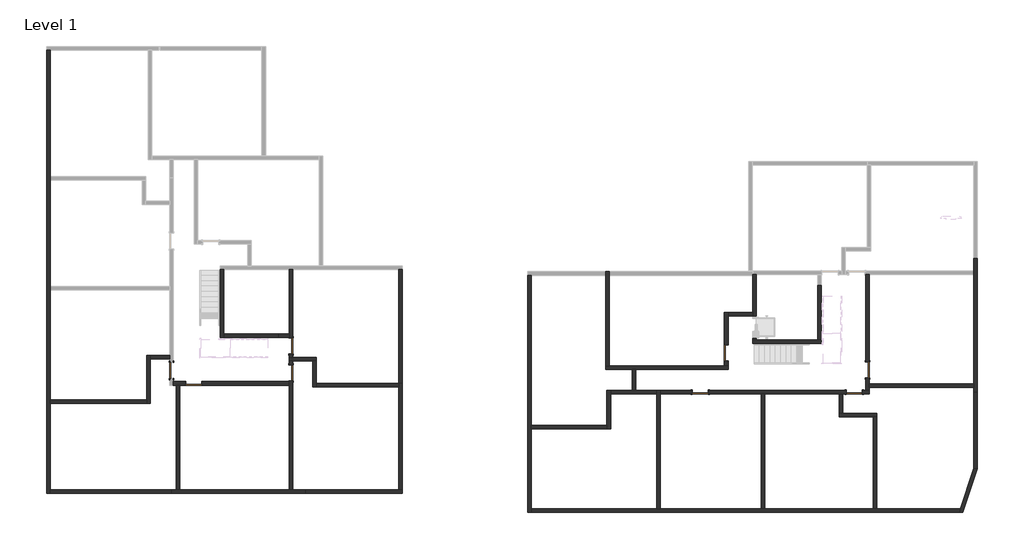
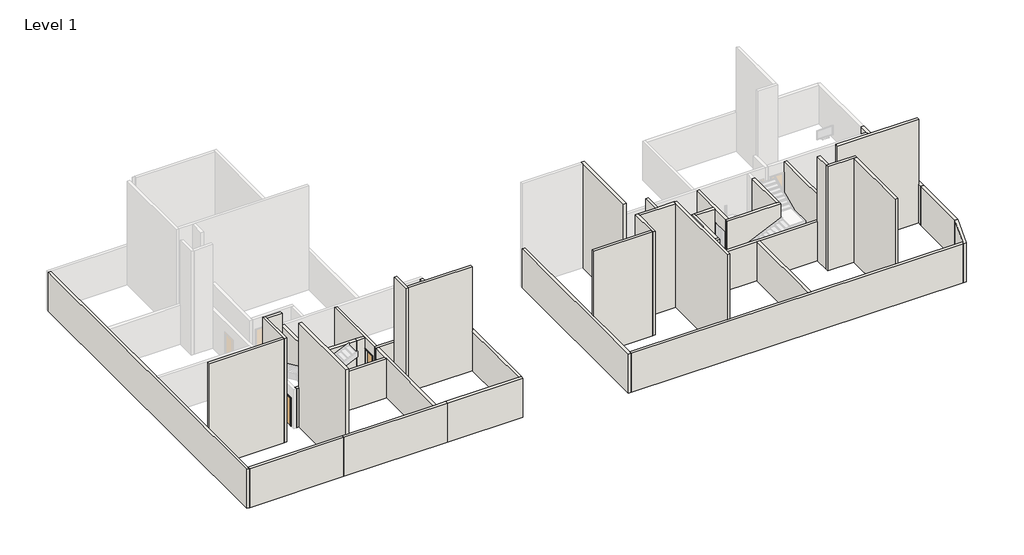
# One storey, part 1 of 2: 43 walls, 8 doors.
"""IFC4 building model written with IfcOpenShell, lengths in millimetres."""

import ifcopenshell
import ifcopenshell.guid

model = None  # the IFC model being written
_history = None  # IfcOwnerHistory: only IFC2X3 demands one
_inside = {}  # id of a spatial element -> (the spatial element, [elements in it])
_under = {}  # id of a project, library or spatial element -> (it, [spatial elements below it])
_declared = {}  # id of a project -> (the project, [libraries it declares])
_typed = {}  # id of a type object -> (the type object, [elements of that type])
_made_of = {}  # id of a material, layer set ... -> (it, [elements and type objects made of it])


def new_model(schema):
    """Start an empty IFC model of exactly this schema.

    Asked for "IFC4X3", IfcOpenShell would pick the latest addendum, in which some entities
    have other attributes; the version numbers below select the first issue.
    IFC2X3 requires an IfcOwnerHistory on every rooted entity: one is made here for all.
    """
    global model, _history
    if schema == "IFC4X3":
        model = ifcopenshell.file(schema_version=(4, 3, 0, 0))
    else:
        model = ifcopenshell.file(schema=schema)
    _inside.clear()
    _under.clear()
    _declared.clear()
    _typed.clear()
    _made_of.clear()
    _history = None
    if model.schema == "IFC2X3":
        org = make("IfcOrganization", Name="unknown")
        user = make(
            "IfcPersonAndOrganization",
            ThePerson=make("IfcPerson", FamilyName="unknown"),
            TheOrganization=org,
        )
        app = make(
            "IfcApplication",
            ApplicationDeveloper=org,
            Version="unknown",
            ApplicationFullName="unknown",
            ApplicationIdentifier="unknown",
        )
        _history = make(
            "IfcOwnerHistory",
            OwningUser=user,
            OwningApplication=app,
            ChangeAction="ADDED",
            CreationDate=0,
        )
    return model


def make(cls, **values):
    """One entity of the class cls with the attributes given. An attribute that is None is left unset."""
    return model.create_entity(
        cls, **{name: value for name, value in values.items() if value is not None}
    )


def rooted(cls, **values):
    """An entity with a GlobalId (a new one), such as an element, a storey or a relation."""
    return make(cls, GlobalId=ifcopenshell.guid.new(), OwnerHistory=_history, **values)


def si_unit(unit_type, name, prefix=None):
    """IfcSIUnit, for example si_unit("LENGTHUNIT", "METRE", prefix="MILLI")."""
    return make("IfcSIUnit", UnitType=unit_type, Prefix=prefix, Name=name)


def assignment(units):
    """IfcUnitAssignment: the units of a project."""
    return None if units is None else make("IfcUnitAssignment", Units=units)


def point(xyz):
    """IfcCartesianPoint."""
    return None if xyz is None else make("IfcCartesianPoint", Coordinates=xyz)


def direction(xyz):
    """IfcDirection."""
    return None if xyz is None else make("IfcDirection", DirectionRatios=xyz)


def frame(location, z_axis=None, x_axis=None):
    """IfcAxis2Placement3D, a coordinate frame: its origin and axes. An axis left out is left unset."""
    return make(
        "IfcAxis2Placement3D",
        Location=point(location),
        Axis=direction(z_axis),
        RefDirection=direction(x_axis),
    )


def origin():
    """The frame at (0, 0, 0) with its axes left unset."""
    return frame((0.0, 0.0, 0.0))


def origin_with_axes():
    """The frame at (0, 0, 0) with the z axis (0, 0, 1) and the x axis (1, 0, 0) written out."""
    return frame((0.0, 0.0, 0.0), z_axis=(0.0, 0.0, 1.0), x_axis=(1.0, 0.0, 0.0))


def place(relative_to, where):
    """IfcLocalPlacement: puts the frame where relative to a parent placement (None: the world)."""
    return make(
        "IfcLocalPlacement", PlacementRelTo=relative_to, RelativePlacement=where
    )


def context(
    kind, dimensions, precision=None, world=None, true_north=None, identifier=None
):
    """IfcGeometricRepresentationContext, for example the 3D "Model" context."""
    return make(
        "IfcGeometricRepresentationContext",
        ContextIdentifier=identifier,
        ContextType=kind,
        CoordinateSpaceDimension=dimensions,
        Precision=precision,
        WorldCoordinateSystem=world,
        TrueNorth=true_north,
    )


def project(units=None, contexts=None):
    """IfcProject with its units and contexts."""
    return rooted(
        "IfcProject",
        Name="project",
        RepresentationContexts=contexts,
        UnitsInContext=assignment(units),
    )


def spatial(cls, under=None, at=None, **own):
    """A site, building, storey or space (cls), placed at a placement, below another one or the project."""
    s = rooted(cls, ObjectPlacement=at, **own)
    if under is not None:
        _under.setdefault(under.id(), (under, []))[1].append(s)
    return s


def polyline(points):
    """IfcPolyline through the points."""
    return make("IfcPolyline", Points=[point(p) for p in points])


def outline(outer, holes=None, kind="AREA"):
    """IfcArbitraryClosedProfileDef: a profile drawn as a closed curve; with holes, ...WithVoids."""
    if holes is None:
        return make("IfcArbitraryClosedProfileDef", ProfileType=kind, OuterCurve=outer)
    return make(
        "IfcArbitraryProfileDefWithVoids",
        ProfileType=kind,
        OuterCurve=outer,
        InnerCurves=holes,
    )


def extrude(swept, where, along, depth):
    """IfcExtrudedAreaSolid: the profile swept, set in the frame where, extruded along a direction by depth."""
    return make(
        "IfcExtrudedAreaSolid",
        SweptArea=swept,
        Position=where,
        ExtrudedDirection=direction(along),
        Depth=depth,
    )


def faces_of(points, faces, orient=None, outer=None):
    """IfcFace entities. A face is a list of loops; a loop is a list of indices into points, from 0.

    orient and outer hold one flag for each loop. By default every Orientation is true, the
    first loop of a face is its IfcFaceOuterBound and the others are IfcFaceBound.
    """
    made = []
    for i, loops in enumerate(faces):
        bounds = []
        for j, loop in enumerate(loops):
            is_outer = j == 0 if outer is None else outer[i][j]
            bounds.append(
                make(
                    "IfcFaceOuterBound" if is_outer else "IfcFaceBound",
                    Bound=make("IfcPolyLoop", Polygon=[points[k] for k in loop]),
                    Orientation=True if orient is None else orient[i][j],
                )
            )
        made.append(make("IfcFace", Bounds=bounds))
    return made


def faceted_brep(points, faces, orient=None, outer=None, voids=None):
    """IfcFacetedBrep: a solid bounded by flat faces; with voids (closed shells), ...WithVoids."""
    shared = [point(p) for p in points]
    hull = make("IfcClosedShell", CfsFaces=faces_of(shared, faces, orient, outer))
    if voids is None:
        return make("IfcFacetedBrep", Outer=hull)
    return make(
        "IfcFacetedBrepWithVoids",
        Outer=hull,
        Voids=[
            make(cls, CfsFaces=faces_of(shared, fs, o, b)) for cls, fs, o, b in voids
        ],
    )


def shape(context_of_items, identifier, shape_type, items):
    """IfcShapeRepresentation: the items that make up one representation, for example the "Body"."""
    return make(
        "IfcShapeRepresentation",
        ContextOfItems=context_of_items,
        RepresentationIdentifier=identifier,
        RepresentationType=shape_type,
        Items=items,
    )


def source(mapping_origin, context_of_items, identifier, shape_type, items):
    """IfcRepresentationMap: a shape defined once, which mapped items show again and again."""
    return make(
        "IfcRepresentationMap",
        MappingOrigin=mapping_origin,
        MappedRepresentation=shape(context_of_items, identifier, shape_type, items),
    )


def transform(
    local_origin,
    x_axis=None,
    y_axis=None,
    z_axis=None,
    scale=None,
    scale2=None,
    scale3=None,
    uniform=True,
):
    """IfcCartesianTransformationOperator3D, or its non-uniform kind. x_axis, y_axis, z_axis: its Axis1, 2, 3."""
    if uniform:
        return make(
            "IfcCartesianTransformationOperator3D",
            Axis1=direction(x_axis),
            Axis2=direction(y_axis),
            LocalOrigin=point(local_origin),
            Scale=scale,
            Axis3=direction(z_axis),
        )
    return make(
        "IfcCartesianTransformationOperator3DnonUniform",
        Axis1=direction(x_axis),
        Axis2=direction(y_axis),
        LocalOrigin=point(local_origin),
        Scale=scale,
        Axis3=direction(z_axis),
        Scale2=scale2,
        Scale3=scale3,
    )


def mapped(mapping_source, mapping_target):
    """IfcMappedItem: shows the shape of a source again, moved by a transform."""
    return make(
        "IfcMappedItem", MappingSource=mapping_source, MappingTarget=mapping_target
    )


def made_of(thing, what):
    """Note that an element or type object is made of a material, layer set ...; save() writes the relation."""
    if what is not None:
        _made_of.setdefault(what.id(), (what, []))[1].append(thing)
    return thing


def element(
    cls,
    number,
    at=None,
    inside=None,
    cuts=None,
    type_object=None,
    material=None,
    context=None,
    identifier="Body",
    shape_type=None,
    held_by="IfcProductDefinitionShape",
    body=None,
    shapes=None,
    **own,
):
    """One element of the class cls, such as IfcWall. Its Tag is "e" and its number.

    at: its placement. inside: the storey or other place that contains it. cuts: it is an
    opening in that element (IfcRelVoidsElement). A single representation is given by context,
    identifier, shape_type and body (its items); several are given by shapes. held_by: the class
    of the entity that holds the representations. save() writes the other relations.
    """
    e = rooted(cls, Tag="e%d" % number, ObjectPlacement=at, **own)
    if body is not None:
        shapes = [shape(context, identifier, shape_type, body)]
    if shapes is not None:
        e.Representation = make(held_by, Representations=shapes)
    if inside is not None:
        _inside.setdefault(inside.id(), (inside, []))[1].append(e)
    if cuts is not None:
        rooted(
            "IfcRelVoidsElement", RelatingBuildingElement=cuts, RelatedOpeningElement=e
        )
    if type_object is not None:
        _typed.setdefault(type_object.id(), (type_object, []))[1].append(e)
    return made_of(e, material)


def aggregate(whole, parts):
    """IfcRelAggregates: a whole, such as a stair, and the parts it consists of."""
    return rooted("IfcRelAggregates", RelatingObject=whole, RelatedObjects=parts)


def save(model, path):
    """Write the relations noted so far, then the file.

    IfcRelAggregates (storeys below a building ...), IfcRelContainedInSpatialStructure (elements
    in a storey), IfcRelDefinesByType, IfcRelAssociatesMaterial and IfcRelDeclares: one each for
    every whole, place, type object, material and project.
    """
    for whole, parts in _under.values():
        aggregate(whole, parts)
    for where, things in _inside.values():
        rooted(
            "IfcRelContainedInSpatialStructure",
            RelatedElements=things,
            RelatingStructure=where,
        )
    for kind, things in _typed.values():
        rooted("IfcRelDefinesByType", RelatedObjects=things, RelatingType=kind)
    for what, things in _made_of.values():
        rooted("IfcRelAssociatesMaterial", RelatedObjects=things, RelatingMaterial=what)
    for by, libraries in _declared.values():
        rooted("IfcRelDeclares", RelatingContext=by, RelatedDefinitions=libraries)
    model.write(path)


def m_single_flush_0915_x_2134mm_727434cd(model_context):
    return source(origin(), model_context, "Body", "SweptSolid", [
        extrude(outline(polyline([(2210.0, -533.5), (0.0, -533.5), (0.0, -457.5), (2134.0, -457.5), (2134.0, 457.5), (0.0, 457.5), (0.0, 533.5), (2210.0, 533.5), (2210.0, -533.5)])), frame((0.0, -125.0, 0.0), z_axis=(0.0, 1.0, 0.0), x_axis=(0.0, 0.0, 1.0)), (0.0, 0.0, 1.0), 25.0),
        extrude(outline(polyline([(2210.0, 533.5), (2210.0, -533.5), (0.0, -533.5), (0.0, -457.5), (2134.0, -457.5), (2134.0, 457.5), (0.0, 457.5), (0.0, 533.5), (2210.0, 533.5)])), frame((0.0, 100.0, 0.0), z_axis=(0.0, 1.0, 0.0), x_axis=(0.0, 0.0, 1.0)), (0.0, 0.0, 1.0), 25.0),
        extrude(outline(polyline([(457.5, -49.0), (457.5, -100.0), (-457.5, -100.0), (-457.5, -49.0), (457.5, -49.0)])), origin_with_axes(), (0.0, 0.0, 1.0), 2134.0),
    ])


def m_single_flush_0915_x_2134mm_6a9e8738(model_context):
    return source(origin(), model_context, "Body", "SweptSolid", [
        extrude(outline(polyline([(2210.0, -533.5), (0.0, -533.5), (0.0, -457.5), (2134.0, -457.5), (2134.0, 457.5), (0.0, 457.5), (0.0, 533.5), (2210.0, 533.5), (2210.0, -533.5)])), frame((0.0, 100.0, 0.0), z_axis=(0.0, 1.0, 0.0), x_axis=(0.0, 0.0, 1.0)), (0.0, 0.0, 1.0), 25.0),
        extrude(outline(polyline([(2210.0, 533.5), (2210.0, -533.5), (0.0, -533.5), (0.0, -457.5), (2134.0, -457.5), (2134.0, 457.5), (0.0, 457.5), (0.0, 533.5), (2210.0, 533.5)])), frame((0.0, -125.0, 0.0), z_axis=(0.0, 1.0, 0.0), x_axis=(0.0, 0.0, 1.0)), (0.0, 0.0, 1.0), 25.0),
        extrude(outline(polyline([(457.5, 49.0), (-457.5, 49.0), (-457.5, 100.0), (457.5, 100.0), (457.5, 49.0)])), origin_with_axes(), (0.0, 0.0, 1.0), 2134.0),
    ])


model = new_model("IFC4")

# Units and contexts
model_context = context("Model", 3, world=origin())
ifc_project = project(units=[si_unit("LENGTHUNIT", "METRE", prefix="MILLI")], contexts=[model_context])

# Site, building, storey
site = spatial("IfcSite", under=ifc_project)
building = spatial("IfcBuilding", under=site)
storey = spatial("IfcBuildingStorey", under=building, Name="Level 1", Elevation=0.0)

# Doors
placement = place(None, origin())
m_single_flush_0915_x_2134mm_shape = m_single_flush_0915_x_2134mm_727434cd(model_context)
element("IfcDoor", 1, ObjectType="M_Single-Flush : 0915 x 2134mm", at=placement, inside=storey, context=model_context, shape_type="MappedRepresentation", body=[
    mapped(m_single_flush_0915_x_2134mm_shape, transform((16070.6041014, -3023.024372, 0.0), x_axis=(0.0, -1.0, 0.0), y_axis=(1.0, 0.0, 0.0), z_axis=(0.0, 0.0, 1.0))),
])
element("IfcDoor", 2, ObjectType="M_Single-Flush : 0915 x 2134mm", at=placement, inside=storey, context=model_context, shape_type="MappedRepresentation", body=[
    mapped(m_single_flush_0915_x_2134mm_shape, transform((-8530.3449834, -4137.6378151, 0.0), x_axis=(0.0, 1.0, 0.0), y_axis=(-1.0, 0.0, 0.0), z_axis=(0.0, 0.0, 1.0))),
])
m_single_flush_0915_x_2134mm_2_shape = m_single_flush_0915_x_2134mm_6a9e8738(model_context)
element("IfcDoor", 3, ObjectType="M_Single-Flush : 0915 x 2134mm", at=placement, inside=storey, context=model_context, shape_type="MappedRepresentation", body=[
    mapped(m_single_flush_0915_x_2134mm_2_shape, transform((14602.336337, -5240.0098119, 0.0), x_axis=(-1.0, 0.0, 0.0), y_axis=(0.0, -1.0, 0.0), z_axis=(0.0, 0.0, 1.0))),
])
element("IfcDoor", 4, ObjectType="M_Single-Flush : 0915 x 2134mm", at=placement, inside=storey, context=model_context, shape_type="MappedRepresentation", body=[
    mapped(m_single_flush_0915_x_2134mm_2_shape, transform((24048.8612349, -3982.5098119, 0.0), x_axis=(0.0, -1.0, 0.0), y_axis=(1.0, 0.0, 0.0), z_axis=(0.0, 0.0, 1.0))),
])
element("IfcDoor", 5, ObjectType="M_Single-Flush : 0915 x 2134mm", at=placement, inside=storey, context=model_context, shape_type="MappedRepresentation", body=[
    mapped(m_single_flush_0915_x_2134mm_2_shape, transform((23308.8612349, -5240.0098119, 0.0), x_axis=(-1.0, 0.0, 0.0), y_axis=(0.0, -1.0, 0.0), z_axis=(0.0, 0.0, 1.0))),
])
element("IfcDoor", 6, ObjectType="M_Single-Flush : 0915 x 2134mm", at=placement, inside=storey, context=model_context, shape_type="MappedRepresentation", body=[
    mapped(m_single_flush_0915_x_2134mm_2_shape, transform((-14032.3304233, -4739.1627129, 0.0), x_axis=(-1.0, 0.0, 0.0), y_axis=(0.0, -1.0, 0.0), z_axis=(0.0, 0.0, 1.0))),
])
element("IfcDoor", 7, ObjectType="M_Single-Flush : 0915 x 2134mm", at=placement, inside=storey, context=model_context, shape_type="MappedRepresentation", body=[
    mapped(m_single_flush_0915_x_2134mm_2_shape, transform((-8530.3449834, -2622.6378151, 0.0), x_axis=(0.0, -1.0, 0.0), y_axis=(1.0, 0.0, 0.0), z_axis=(0.0, 0.0, 1.0))),
])
element("IfcDoor", 8, ObjectType="M_Single-Flush : 0915 x 2134mm", at=placement, inside=storey, context=model_context, shape_type="MappedRepresentation", body=[
    mapped(m_single_flush_0915_x_2134mm_2_shape, transform((-15289.8304233, -3999.1627129, 0.0), x_axis=(0.0, 1.0, 0.0), y_axis=(-1.0, 0.0, 0.0), z_axis=(0.0, 0.0, 1.0))),
])

# Walls
element("IfcWall", 9, ObjectType="Generic - 200mm", at=placement, inside=storey, context=model_context, shape_type="Brep", body=[
    faceted_brep([(30068.8612349, 2319.475628, 0.0), (30068.8612349, 1619.475628, 0.0), (30068.8612349, 1419.475628, 0.0), (30068.8612349, -4760.0098119, 0.0), (30068.8612349, -4960.0098119, 0.0), (30068.8612349, -5240.0098119, 0.0), (30068.8612349, -5240.0098119, 3000.0), (30068.8612349, 1419.475628, 3000.0), (30068.8612349, 1619.475628, 3000.0), (30068.8612349, 2319.475628, 3000.0), (30268.8612349, 2319.475628, 0.0), (30268.8612349, 2319.475628, 3000.0), (30268.8612349, -5240.0098119, 3000.0), (30268.8612349, -5240.0098119, 0.0), (30268.3425199, 2319.475628, 0.0), (30069.3799498, -5240.0098119, 0.0), (30069.3799498, -5240.0098119, 3000.0), (30268.3425199, 2319.475628, 3000.0)], [[[0, 1, 2, 3, 4, 5, 6, 7, 8, 9]], [[10, 11, 12, 13]], [[5, 4, 3, 2, 1, 0, 14, 10, 13, 15]], [[6, 5, 15, 13, 12, 16]], [[9, 8, 7, 6, 16, 12, 11, 17]], [[0, 9, 17, 11, 10, 14]]]),
])
element("IfcWall", 10, ObjectType="Generic - 200mm", at=placement, inside=storey, context=model_context, shape_type="Brep", body=[
    faceted_brep([(30069.3799498, -5240.0098119, 0.0), (30069.3799498, -9543.0251929, 0.0), (30069.3799498, -9543.0251929, 3000.0), (30069.3799498, -5240.0098119, 3000.0), (30269.3799498, -5240.0098119, 0.0), (30269.3799498, -5240.0098119, 3000.0), (30269.3799498, -9575.863443, 3000.0), (30269.3799498, -9575.863443, 0.0), (30268.8612349, -5240.0098119, 0.0), (30268.8612349, -5240.0098119, 3000.0)], [[[0, 1, 2, 3]], [[4, 5, 6, 7]], [[1, 0, 8, 4, 7]], [[3, 2, 6, 5, 9]], [[0, 3, 9, 5, 4, 8]], [[2, 1, 7, 6]]]),
])
element("IfcWall", 11, ObjectType="Generic - 200mm", at=placement, inside=storey, context=model_context, shape_type="Brep", body=[
    faceted_brep([(21449.836337, -2276.2808257, 0.0), (21249.836337, -2276.2808257, 0.0), (17770.6041014, -2276.2808257, 0.0), (17570.6041014, -2276.2808257, 0.0), (17570.6041014, -2276.2808257, 3000.0), (17770.6041014, -2276.2808257, 3000.0), (21249.836337, -2276.2808257, 3000.0), (21449.836337, -2276.2808257, 3000.0), (21449.836337, -2476.2808257, 0.0), (21449.836337, -2476.2808257, 3000.0), (17570.6041014, -2476.2808257, 3000.0), (17570.6041014, -2476.2808257, 0.0)], [[[0, 1, 2, 3, 4, 5, 6, 7]], [[8, 9, 10, 11]], [[3, 2, 1, 0, 8, 11]], [[7, 6, 5, 4, 10, 9]], [[0, 7, 9, 8]], [[4, 3, 11, 10]]]),
])
element("IfcWall", 12, ObjectType="Generic - 200mm", at=placement, inside=storey, context=model_context, shape_type="SweptSolid", body=[
    extrude(outline(polyline([(18259.836337, -5340.0098119), (18259.836337, -11836.6907835), (18059.836337, -11836.6907835), (18059.836337, -5340.0098119), (18259.836337, -5340.0098119)])), origin_with_axes(), (0.0, 0.0, 1.0), 3000.0),
])
element("IfcWall", 13, ObjectType="Generic - 200mm", at=placement, inside=storey, context=model_context, shape_type="Brep", body=[
    faceted_brep([(29295.3124022, -11836.6907835, 0.0), (24588.8612349, -11836.6907835, 0.0), (24388.8612349, -11836.6907835, 0.0), (18259.836337, -11836.6907835, 0.0), (18059.836337, -11836.6907835, 0.0), (12342.1281129, -11836.6907835, 0.0), (12142.1281129, -11836.6907835, 0.0), (5043.716007, -11836.6907835, 0.0), (5043.716007, -11836.6907835, 3000.0), (18059.836337, -11836.6907835, 3000.0), (18259.836337, -11836.6907835, 3000.0), (29295.3124022, -11836.6907835, 3000.0), (29227.8162902, -12036.6907835, 0.0), (29227.8162902, -12036.6907835, 3000.0), (5043.716007, -12036.6907835, 3000.0), (5043.716007, -12036.6907835, 0.0)], [[[0, 1, 2, 3, 4, 5, 6, 7, 8, 9, 10, 11]], [[12, 13, 14, 15]], [[7, 6, 5, 4, 3, 2, 1, 0, 12, 15]], [[11, 10, 9, 8, 14, 13]], [[0, 11, 13, 12]], [[8, 7, 15, 14]]]),
])
element("IfcWall", 14, ObjectType="Generic - 200mm", at=placement, inside=storey, context=model_context, shape_type="Brep", body=[
    faceted_brep([(30069.3799498, -9543.0251929, 0.0), (29295.3124022, -11836.6907835, 0.0), (29227.8162902, -12036.6907835, 0.0), (29227.8162902, -12036.6907835, 3000.0), (29295.3124022, -11836.6907835, 3000.0), (30069.3799498, -9543.0251929, 3000.0), (30269.3799498, -9575.863443, 0.0), (30269.3799498, -9575.863443, 3000.0), (29438.8985612, -12036.6907835, 3000.0), (29438.8985612, -12036.6907835, 0.0)], [[[0, 1, 2, 3, 4, 5]], [[6, 7, 8, 9]], [[2, 1, 0, 6, 9]], [[5, 4, 3, 8, 7]], [[0, 5, 7, 6]], [[3, 2, 9, 8]]]),
])
element("IfcWall", 15, ObjectType="Generic - 200mm", at=placement, inside=storey, context=model_context, shape_type="Brep", body=[
    faceted_brep([(22851.3612349, -5140.0098119, 2134.0), (22851.3612349, -5140.0098119, 0.0), (15059.836337, -5140.0098119, 0.0), (15059.836337, -5140.0098119, 2134.0), (14144.836337, -5140.0098119, 2134.0), (14144.836337, -5140.0098119, 0.0), (12342.1281129, -5140.0098119, 0.0), (12342.1281129, -5140.0098119, 3000.0), (23948.8612349, -5140.0098119, 3000.0), (24148.8612349, -5140.0098119, 3000.0), (24163.3998354, -5140.0098119, 3000.0), (24163.3998354, -5140.0098119, 0.0), (24148.8612349, -5140.0098119, 0.0), (23948.8612349, -5140.0098119, 0.0), (23766.3612349, -5140.0098119, 0.0), (23766.3612349, -5140.0098119, 2134.0), (15059.836337, -5340.0098119, 0.0), (18059.836337, -5340.0098119, 0.0), (18259.836337, -5340.0098119, 0.0), (22468.8612349, -5340.0098119, 0.0), (22668.8612349, -5340.0098119, 0.0), (22851.3612349, -5340.0098119, 0.0), (22851.3612349, -5340.0098119, 2134.0), (23766.3612349, -5340.0098119, 2134.0), (23766.3612349, -5340.0098119, 0.0), (24163.3998354, -5340.0098119, 0.0), (24163.3998354, -5340.0098119, 3000.0), (18259.836337, -5340.0098119, 3000.0), (18059.836337, -5340.0098119, 3000.0), (12342.1281129, -5340.0098119, 3000.0), (12342.1281129, -5340.0098119, 0.0), (14144.836337, -5340.0098119, 0.0), (14144.836337, -5340.0098119, 2134.0), (15059.836337, -5340.0098119, 2134.0)], [[[0, 1, 2, 3, 4, 5, 6, 7, 8, 9, 10, 11, 12, 13, 14, 15]], [[16, 17, 18, 19, 20, 21, 22, 23, 24, 25, 26, 27, 28, 29, 30, 31, 32, 33]], [[30, 6, 5, 31]], [[2, 1, 21, 20, 19, 18, 17, 16]], [[14, 13, 12, 11, 25, 24]], [[10, 9, 8, 7, 29, 28, 27, 26]], [[11, 10, 26, 25]], [[4, 32, 31, 5]], [[33, 3, 2, 16]], [[3, 33, 32, 4]], [[22, 21, 1, 0]], [[23, 22, 0, 15]], [[24, 23, 15, 14]], [[7, 6, 30, 29]]]),
])
element("IfcWall", 16, ObjectType="Generic - 200mm", at=placement, inside=storey, context=model_context, shape_type="Brep", body=[
    faceted_brep([(4843.716007, 1379.9901881, 0.0), (4843.716007, -12036.6907835, 0.0), (4843.716007, -12036.6907835, 3000.0), (4843.716007, 1379.9901881, 3000.0), (5043.716007, 1379.9901881, 0.0), (5043.716007, 1379.9901881, 3000.0), (5043.716007, -11836.6907835, 3000.0), (5043.716007, -12036.6907835, 3000.0), (5043.716007, -12036.6907835, 0.0), (5043.716007, -11836.6907835, 0.0), (5043.716007, -7320.0098119, 0.0), (5043.716007, -7120.0098119, 0.0)], [[[0, 1, 2, 3]], [[4, 5, 6, 7, 8, 9, 10, 11]], [[1, 0, 4, 11, 10, 9, 8]], [[3, 2, 7, 6, 5]], [[2, 1, 8, 7]], [[0, 3, 5, 4]]]),
])
element("IfcWall", 17, ObjectType="Generic - 200mm", at=placement, inside=storey, context=model_context, shape_type="Brep", body=[
    faceted_brep([(24148.8612349, 1419.475628, 3000.0), (24148.8612349, -5140.0098119, 3000.0), (24148.8612349, -5140.0098119, 0.0), (24148.8612349, -4960.0098119, 0.0), (24148.8612349, -4760.0098119, 0.0), (24148.8612349, -4440.0098119, 0.0), (24148.8612349, -4440.0098119, 2134.0), (24148.8612349, -3525.0098119, 2134.0), (24148.8612349, -3525.0098119, 0.0), (24148.8612349, 1419.475628, 0.0), (23948.8612349, -5140.0098119, 3000.0), (23948.8612349, 1419.475628, 3000.0), (23948.8612349, 1419.475628, 0.0), (23948.8612349, -3525.0098119, 0.0), (23948.8612349, -3525.0098119, 2134.0), (23948.8612349, -4440.0098119, 2134.0), (23948.8612349, -4440.0098119, 0.0), (23948.8612349, -5140.0098119, 0.0)], [[[0, 1, 2, 3, 4, 5, 6, 7, 8, 9]], [[10, 11, 12, 13, 14, 15, 16, 17]], [[12, 9, 8, 13]], [[2, 17, 16, 5, 4, 3]], [[1, 0, 11, 10]], [[0, 9, 12, 11]], [[15, 6, 5, 16]], [[7, 14, 13, 8]], [[14, 7, 6, 15]], [[2, 1, 10, 17]]]),
])
element("IfcWall", 18, ObjectType="Generic - 200mm", at=placement, inside=storey, context=model_context, shape_type="SweptSolid", body=[
    extrude(outline(polyline([(21249.836337, -2276.2808257), (21249.836337, 799.475628), (21449.836337, 799.475628), (21449.836337, -2276.2808257), (21249.836337, -2276.2808257)])), origin_with_axes(), (0.0, 0.0, 1.0), 3000.0),
])
element("IfcWall", 19, ObjectType="Generic - 200mm", at=placement, inside=storey, context=model_context, shape_type="Brep", body=[
    faceted_brep([(17570.6041014, -2276.2808257, 3000.0), (17570.6041014, -920.524372, 3000.0), (17570.6041014, -720.524372, 3000.0), (17570.6041014, 1379.475628, 3000.0), (17570.6041014, 1419.475628, 3000.0), (17570.6041014, 1419.475628, 0.0), (17570.6041014, 1379.475628, 0.0), (17570.6041014, -720.524372, 0.0), (17570.6041014, -920.524372, 0.0), (17570.6041014, -926.2808257, 0.0), (17570.6041014, -926.2808257, 2000.0), (17570.6041014, -2181.2876228, 2000.0), (17570.6041014, -2181.2876228, 0.0), (17570.6041014, -2276.2808257, 0.0), (17770.6041014, 1419.475628, 3000.0), (17770.6041014, -2276.2808257, 3000.0), (17770.6041014, -2276.2808257, 0.0), (17770.6041014, -2181.2876228, 0.0), (17770.6041014, -2181.2876228, 2000.0), (17770.6041014, -926.2808257, 2000.0), (17770.6041014, -926.2808257, 0.0), (17770.6041014, 1419.475628, 0.0)], [[[0, 1, 2, 3, 4, 5, 6, 7, 8, 9, 10, 11, 12, 13]], [[14, 15, 16, 17, 18, 19, 20, 21]], [[16, 13, 12, 17]], [[5, 21, 20, 9, 8, 7, 6]], [[4, 3, 2, 1, 0, 15, 14]], [[0, 13, 16, 15]], [[5, 4, 14, 21]], [[11, 18, 17, 12]], [[19, 10, 9, 20]], [[10, 19, 18, 11]]]),
])
element("IfcWall", 20, ObjectType="Generic - 200mm", at=placement, inside=storey, context=model_context, shape_type="Brep", body=[
    faceted_brep([(9268.8612349, -3940.0098119, 0.0), (10768.8612349, -3940.0098119, 0.0), (10968.8612349, -3940.0098119, 0.0), (16170.6041014, -3940.0098119, 0.0), (16170.6041014, -3940.0098119, 3000.0), (9268.8612349, -3940.0098119, 3000.0), (9268.8612349, -3740.0098119, 0.0), (9268.8612349, -3740.0098119, 3000.0), (15970.6041014, -3740.0098119, 3000.0), (16170.6041014, -3740.0098119, 3000.0), (16170.6041014, -3740.0098119, 0.0), (15970.6041014, -3740.0098119, 0.0), (9468.8612349, -3740.0098119, 0.0)], [[[0, 1, 2, 3, 4, 5]], [[6, 7, 8, 9, 10, 11, 12]], [[3, 2, 1, 0, 6, 12, 11, 10]], [[5, 4, 9, 8, 7]], [[4, 3, 10, 9]], [[0, 5, 7, 6]]]),
])
element("IfcWall", 21, ObjectType="Generic - 200mm", at=placement, inside=storey, context=model_context, shape_type="Brep", body=[
    faceted_brep([(16170.6041014, -720.524372, 3000.0), (16170.6041014, -920.524372, 3000.0), (16170.6041014, -3740.0098119, 3000.0), (16170.6041014, -3740.0098119, 0.0), (16170.6041014, -3480.524372, 0.0), (16170.6041014, -3480.524372, 2134.0), (16170.6041014, -2565.524372, 2134.0), (16170.6041014, -2565.524372, 0.0), (16170.6041014, -920.524372, 0.0), (16170.6041014, -720.524372, 0.0), (15970.6041014, -3740.0098119, 3000.0), (15970.6041014, -720.524372, 3000.0), (15970.6041014, -720.524372, 0.0), (15970.6041014, -2565.524372, 0.0), (15970.6041014, -2565.524372, 2134.0), (15970.6041014, -3480.524372, 2134.0), (15970.6041014, -3480.524372, 0.0), (15970.6041014, -3740.0098119, 0.0)], [[[0, 1, 2, 3, 4, 5, 6, 7, 8, 9]], [[10, 11, 12, 13, 14, 15, 16, 17]], [[3, 17, 16, 4]], [[12, 9, 8, 7, 13]], [[2, 1, 0, 11, 10]], [[3, 2, 10, 17]], [[0, 9, 12, 11]], [[15, 5, 4, 16]], [[6, 14, 13, 7]], [[14, 6, 5, 15]]]),
])
element("IfcWall", 22, ObjectType="Generic - 200mm", at=placement, inside=storey, context=model_context, shape_type="SweptSolid", body=[
    extrude(outline(polyline([(17570.6041014, -920.524372), (16170.6041014, -920.524372), (16170.6041014, -720.524372), (17570.6041014, -720.524372), (17570.6041014, -920.524372)])), origin_with_axes(), (0.0, 0.0, 1.0), 3000.0),
])
element("IfcWall", 23, ObjectType="Generic - 200mm", at=placement, inside=storey, context=model_context, shape_type="Brep", body=[
    faceted_brep([(22468.8612349, -6641.2808257, 0.0), (24388.8612349, -6641.2808257, 0.0), (24588.8612349, -6641.2808257, 0.0), (24588.8612349, -6641.2808257, 8000.0), (24388.8612349, -6641.2808257, 8000.0), (22468.8612349, -6641.2808257, 8000.0), (22468.8612349, -6441.2808257, 0.0), (22468.8612349, -6441.2808257, 8000.0), (22668.8612349, -6441.2808257, 8000.0), (24588.8612349, -6441.2808257, 8000.0), (24588.8612349, -6441.2808257, 0.0), (22668.8612349, -6441.2808257, 0.0)], [[[0, 1, 2, 3, 4, 5]], [[6, 7, 8, 9, 10, 11]], [[2, 1, 0, 6, 11, 10]], [[5, 4, 3, 9, 8, 7]], [[3, 2, 10, 9]], [[0, 5, 7, 6]]]),
])
element("IfcWall", 24, ObjectType="Generic - 200mm", at=placement, inside=storey, context=model_context, shape_type="SweptSolid", body=[
    extrude(outline(polyline([(24388.8612349, -11836.6907835), (24388.8612349, -6641.2808257), (24588.8612349, -6641.2808257), (24588.8612349, -11836.6907835), (24388.8612349, -11836.6907835)])), origin_with_axes(), (0.0, 0.0, 1.0), 8000.0),
])
element("IfcWall", 25, ObjectType="Generic - 200mm", at=placement, inside=storey, context=model_context, shape_type="SweptSolid", body=[
    extrude(outline(polyline([(22668.8612349, -5340.0098119), (22668.8612349, -6441.2808257), (22468.8612349, -6441.2808257), (22468.8612349, -5340.0098119), (22668.8612349, -5340.0098119)])), origin_with_axes(), (0.0, 0.0, 1.0), 8000.0),
])
element("IfcWall", 26, ObjectType="Generic - 200mm", at=placement, inside=storey, context=model_context, shape_type="SweptSolid", body=[
    extrude(outline(polyline([(30068.8612349, -4960.0098119), (24148.8612349, -4960.0098119), (24148.8612349, -4760.0098119), (30068.8612349, -4760.0098119), (30068.8612349, -4960.0098119)])), origin_with_axes(), (0.0, 0.0, 1.0), 8000.0),
])
element("IfcWall", 27, ObjectType="Generic - 200mm", at=placement, inside=storey, context=model_context, shape_type="Brep", body=[
    faceted_brep([(9268.8612349, 1579.9901881, 0.0), (9268.8612349, 1379.9901881, 0.0), (9268.8612349, -3740.0098119, 0.0), (9268.8612349, -3740.0098119, 3000.0), (9268.8612349, -3740.0098119, 8000.0), (9268.8612349, 1379.9901881, 8000.0), (9268.8612349, 1579.9901881, 8000.0), (9468.8612349, 1579.9901881, 0.0), (9468.8612349, 1579.9901881, 8000.0), (9468.8612349, -3740.0098119, 8000.0), (9468.8612349, -3740.0098119, 0.0), (9468.8612349, 1379.475628, 0.0), (9468.8612349, 1579.475628, 0.0)], [[[0, 1, 2, 3, 4, 5, 6]], [[7, 8, 9, 10, 11, 12]], [[2, 1, 0, 7, 12, 11, 10]], [[6, 5, 4, 9, 8]], [[4, 3, 2, 10, 9]], [[0, 6, 8, 7]]]),
])
element("IfcWall", 28, ObjectType="Generic - 200mm", at=placement, inside=storey, context=model_context, shape_type="SweptSolid", body=[
    extrude(outline(polyline([(5043.716007, -7120.0098119), (9328.8612349, -7120.0098119), (9328.8612349, -7320.0098119), (5043.716007, -7320.0098119), (5043.716007, -7120.0098119)])), origin_with_axes(), (0.0, 0.0, 1.0), 8000.0),
])
element("IfcWall", 29, ObjectType="Generic - 200mm", at=placement, inside=storey, context=model_context, shape_type="Brep", body=[
    faceted_brep([(-2430.3449834, -4740.1378151, 0.0), (-2430.3449834, -4940.1378151, 0.0), (-2430.3449834, -10758.643998, 0.0), (-2430.3449834, -10758.643998, 3000.0), (-2430.3449834, -4740.1378151, 3000.0), (-2230.3449834, -4740.1378151, 0.0), (-2230.3449834, -4740.1378151, 3000.0), (-2230.3449834, -10758.643998, 3000.0), (-2230.3449834, -10758.643998, 0.0)], [[[0, 1, 2, 3, 4]], [[5, 6, 7, 8]], [[2, 1, 0, 5, 8]], [[4, 3, 7, 6]], [[3, 2, 8, 7]], [[0, 4, 6, 5]]]),
])
element("IfcWall", 30, ObjectType="Generic - 200mm", at=placement, inside=storey, context=model_context, shape_type="Brep", body=[
    faceted_brep([(-2230.3449834, -10758.643998, 0.0), (-2430.3449834, -10758.643998, 0.0), (-7730.3449834, -10758.643998, 0.0), (-7730.3449834, -10758.643998, 3000.0), (-2430.3449834, -10758.643998, 3000.0), (-2230.3449834, -10758.643998, 3000.0), (-2230.3449834, -10958.643998, 0.0), (-2230.3449834, -10958.643998, 3000.0), (-7730.3449834, -10958.643998, 3000.0), (-7730.3449834, -10958.643998, 0.0), (-7730.3449834, -10759.1627129, 0.0), (-7730.3449834, -10759.1627129, 3000.0)], [[[0, 1, 2, 3, 4, 5]], [[6, 7, 8, 9]], [[2, 1, 0, 6, 9, 10]], [[3, 2, 10, 9, 8, 11]], [[5, 4, 3, 11, 8, 7]], [[0, 5, 7, 6]]]),
])
element("IfcWall", 31, ObjectType="Generic - 200mm", at=placement, inside=storey, context=model_context, shape_type="Brep", body=[
    faceted_brep([(-7730.3449834, -10759.1627129, 0.0), (-8430.3449834, -10759.1627129, 0.0), (-8630.3449834, -10759.1627129, 0.0), (-14809.8304233, -10759.1627129, 0.0), (-15009.8304233, -10759.1627129, 0.0), (-15289.8304233, -10759.1627129, 0.0), (-15289.8304233, -10759.1627129, 3000.0), (-8630.3449834, -10759.1627129, 3000.0), (-8430.3449834, -10759.1627129, 3000.0), (-7730.3449834, -10759.1627129, 3000.0), (-7730.3449834, -10959.1627129, 0.0), (-7730.3449834, -10959.1627129, 3000.0), (-15289.8304233, -10959.1627129, 3000.0), (-15289.8304233, -10959.1627129, 0.0), (-7730.3449834, -10958.643998, 0.0), (-15289.8304233, -10759.6814279, 0.0), (-15289.8304233, -10759.6814279, 3000.0), (-7730.3449834, -10958.643998, 3000.0)], [[[0, 1, 2, 3, 4, 5, 6, 7, 8, 9]], [[10, 11, 12, 13]], [[5, 4, 3, 2, 1, 0, 14, 10, 13, 15]], [[6, 5, 15, 13, 12, 16]], [[9, 8, 7, 6, 16, 12, 11, 17]], [[0, 9, 17, 11, 10, 14]]]),
])
element("IfcWall", 32, ObjectType="Generic - 200mm", at=placement, inside=storey, context=model_context, shape_type="Brep", body=[
    faceted_brep([(-15289.8304233, -10759.6814279, 0.0), (-22146.5113948, -10759.6814279, 0.0), (-22146.5113948, -10759.6814279, 3000.0), (-15289.8304233, -10759.6814279, 3000.0), (-15289.8304233, -10959.6814279, 0.0), (-15289.8304233, -10959.6814279, 3000.0), (-22146.5113948, -10959.6814279, 3000.0), (-22146.5113948, -10959.6814279, 0.0), (-15289.8304233, -10959.1627129, 0.0), (-15289.8304233, -10959.1627129, 3000.0)], [[[0, 1, 2, 3]], [[4, 5, 6, 7]], [[1, 0, 8, 4, 7]], [[3, 2, 6, 5, 9]], [[0, 3, 9, 5, 4, 8]], [[2, 1, 7, 6]]]),
])
element("IfcWall", 33, ObjectType="Generic - 200mm", at=placement, inside=storey, context=model_context, shape_type="Brep", body=[
    faceted_brep([(-12326.101437, -2140.1378151, 0.0), (-12326.101437, -1940.1378151, 0.0), (-12326.101437, 1699.0944206, 0.0), (-12326.101437, 1699.0944206, 3000.0), (-12326.101437, -1940.1378151, 3000.0), (-12326.101437, -2140.1378151, 3000.0), (-12526.101437, -2140.1378151, 0.0), (-12526.101437, -2140.1378151, 3000.0), (-12526.101437, 1699.0944206, 3000.0), (-12526.101437, 1699.0944206, 0.0)], [[[0, 1, 2, 3, 4, 5]], [[6, 7, 8, 9]], [[2, 1, 0, 6, 9]], [[3, 2, 9, 8]], [[5, 4, 3, 8, 7]], [[0, 5, 7, 6]]]),
])
element("IfcWall", 34, ObjectType="Generic - 200mm", at=placement, inside=storey, context=model_context, shape_type="Brep", body=[
    faceted_brep([(-22146.5113948, -10959.6814279, 0.0), (-22146.5113948, -10759.6814279, 0.0), (-22146.5113948, -5879.1627129, 0.0), (-22146.5113948, -5679.1627129, 0.0), (-22146.5113948, 549.8621849, 0.0), (-22146.5113948, 749.8621849, 0.0), (-22146.5113948, 6769.8621849, 0.0), (-22146.5113948, 6969.8621849, 0.0), (-22146.5113948, 14109.8621849, 0.0), (-22146.5113948, 14109.8621849, 3000.0), (-22146.5113948, 6969.8621849, 3000.0), (-22146.5113948, 6769.8621849, 3000.0), (-22146.5113948, 749.8621849, 3000.0), (-22146.5113948, 549.8621849, 3000.0), (-22146.5113948, -10759.6814279, 3000.0), (-22146.5113948, -10959.6814279, 3000.0), (-22346.5113948, -10959.6814279, 0.0), (-22346.5113948, -10959.6814279, 3000.0), (-22346.5113948, 14109.8621849, 3000.0), (-22346.5113948, 14109.8621849, 0.0)], [[[0, 1, 2, 3, 4, 5, 6, 7, 8, 9, 10, 11, 12, 13, 14, 15]], [[16, 17, 18, 19]], [[8, 7, 6, 5, 4, 3, 2, 1, 0, 16, 19]], [[15, 14, 13, 12, 11, 10, 9, 18, 17]], [[9, 8, 19, 18]], [[0, 15, 17, 16]]]),
])
element("IfcWall", 35, ObjectType="Generic - 200mm", at=placement, inside=storey, context=model_context, shape_type="Brep", body=[
    faceted_brep([(-8630.3449834, -4839.1627129, 3000.0), (-15189.8304233, -4839.1627129, 3000.0), (-15189.8304233, -4839.1627129, 0.0), (-15009.8304233, -4839.1627129, 0.0), (-14809.8304233, -4839.1627129, 0.0), (-14489.8304233, -4839.1627129, 0.0), (-14489.8304233, -4839.1627129, 2134.0), (-13574.8304233, -4839.1627129, 2134.0), (-13574.8304233, -4839.1627129, 0.0), (-8630.3449834, -4839.1627129, 0.0), (-15189.8304233, -4639.1627129, 3000.0), (-8630.3449834, -4639.1627129, 3000.0), (-8630.3449834, -4639.1627129, 0.0), (-13574.8304233, -4639.1627129, 0.0), (-13574.8304233, -4639.1627129, 2134.0), (-14489.8304233, -4639.1627129, 2134.0), (-14489.8304233, -4639.1627129, 0.0), (-15189.8304233, -4639.1627129, 0.0)], [[[0, 1, 2, 3, 4, 5, 6, 7, 8, 9]], [[10, 11, 12, 13, 14, 15, 16, 17]], [[12, 9, 8, 13]], [[2, 17, 16, 5, 4, 3]], [[1, 0, 11, 10]], [[0, 9, 12, 11]], [[15, 6, 5, 16]], [[7, 14, 13, 8]], [[14, 7, 6, 15]], [[2, 1, 10, 17]]]),
])
element("IfcWall", 36, ObjectType="Generic - 200mm", at=placement, inside=storey, context=model_context, shape_type="SweptSolid", body=[
    extrude(outline(polyline([(-12326.101437, -1940.1378151), (-9250.3449834, -1940.1378151), (-9250.3449834, -2140.1378151), (-12326.101437, -2140.1378151), (-12326.101437, -1940.1378151)])), origin_with_axes(), (0.0, 0.0, 1.0), 3000.0),
])
element("IfcWall", 37, ObjectType="Generic - 200mm", at=placement, inside=storey, context=model_context, shape_type="SweptSolid", body=[
    extrude(outline(polyline([(-8630.3449834, -2140.1378151), (-9250.3449834, -2140.1378151), (-9250.3449834, -1940.1378151), (-8630.3449834, -1940.1378151), (-8630.3449834, -2140.1378151)])), origin_with_axes(), (0.0, 0.0, 1.0), 3000.0),
])
element("IfcWall", 38, ObjectType="Generic - 200mm", at=placement, inside=storey, context=model_context, shape_type="SweptSolid", body=[
    extrude(outline(polyline([(-2430.3449834, -4740.1378151), (-2430.3449834, 1700.8372871), (-2230.3449834, 1700.8372871), (-2230.3449834, -4740.1378151), (-2430.3449834, -4740.1378151)])), origin_with_axes(), (0.0, 0.0, 1.0), 3000.0),
])
element("IfcWall", 39, ObjectType="Generic - 200mm", at=placement, inside=storey, context=model_context, shape_type="Brep", body=[
    faceted_brep([(-8630.3449834, -3480.1378151, 0.0), (-8430.3449834, -3480.1378151, 0.0), (-7295.3449834, -3480.1378151, 0.0), (-7095.3449834, -3480.1378151, 0.0), (-7095.3449834, -3480.1378151, 3000.0), (-8430.3449834, -3480.1378151, 3000.0), (-8630.3449834, -3480.1378151, 3000.0), (-8630.3449834, -3280.1378151, 0.0), (-8630.3449834, -3280.1378151, 3000.0), (-8430.3449834, -3280.1378151, 3000.0), (-7095.3449834, -3280.1378151, 3000.0), (-7095.3449834, -3280.1378151, 0.0), (-8430.3449834, -3280.1378151, 0.0)], [[[0, 1, 2, 3, 4, 5, 6]], [[7, 8, 9, 10, 11, 12]], [[3, 2, 1, 0, 7, 12, 11]], [[6, 5, 4, 10, 9, 8]], [[0, 6, 8, 7]], [[4, 3, 11, 10]]]),
])
element("IfcWall", 40, ObjectType="Generic - 200mm", at=placement, inside=storey, context=model_context, shape_type="Brep", body=[
    faceted_brep([(-8630.3449834, -10759.1627129, 3000.0), (-8630.3449834, -4839.1627129, 3000.0), (-8630.3449834, -4639.1627129, 3000.0), (-8630.3449834, -3480.1378151, 3000.0), (-8630.3449834, -3480.1378151, 0.0), (-8630.3449834, -3680.1378151, 0.0), (-8630.3449834, -3680.1378151, 2134.0), (-8630.3449834, -4595.1378151, 2134.0), (-8630.3449834, -4595.1378151, 0.0), (-8630.3449834, -4639.1627129, 0.0), (-8630.3449834, -4839.1627129, 0.0), (-8630.3449834, -10759.1627129, 0.0), (-8430.3449834, -3480.1378151, 3000.0), (-8430.3449834, -10759.1627129, 3000.0), (-8430.3449834, -10759.1627129, 0.0), (-8430.3449834, -4595.1378151, 0.0), (-8430.3449834, -4595.1378151, 2134.0), (-8430.3449834, -3680.1378151, 2134.0), (-8430.3449834, -3680.1378151, 0.0), (-8430.3449834, -3480.1378151, 0.0)], [[[0, 1, 2, 3, 4, 5, 6, 7, 8, 9, 10, 11]], [[12, 13, 14, 15, 16, 17, 18, 19]], [[14, 11, 10, 9, 8, 15]], [[4, 19, 18, 5]], [[3, 2, 1, 0, 13, 12]], [[0, 11, 14, 13]], [[4, 3, 12, 19]], [[17, 6, 5, 18]], [[7, 16, 15, 8]], [[16, 7, 6, 17]]]),
])
element("IfcWall", 41, ObjectType="Generic - 200mm", at=placement, inside=storey, context=model_context, shape_type="Brep", body=[
    faceted_brep([(-8430.3449834, 1700.8372871, 3000.0), (-8430.3449834, -3280.1378151, 3000.0), (-8430.3449834, -3280.1378151, 0.0), (-8430.3449834, -3080.1378151, 0.0), (-8430.3449834, -3080.1378151, 2134.0), (-8430.3449834, -2165.1378151, 2134.0), (-8430.3449834, -2165.1378151, 0.0), (-8430.3449834, 1700.8372871, 0.0), (-8630.3449834, -3280.1378151, 3000.0), (-8630.3449834, -2140.1378151, 3000.0), (-8630.3449834, -1940.1378151, 3000.0), (-8630.3449834, 1700.8372871, 3000.0), (-8630.3449834, 1700.8372871, 0.0), (-8630.3449834, -1940.1378151, 0.0), (-8630.3449834, -2140.1378151, 0.0), (-8630.3449834, -2165.1378151, 0.0), (-8630.3449834, -2165.1378151, 2134.0), (-8630.3449834, -3080.1378151, 2134.0), (-8630.3449834, -3080.1378151, 0.0), (-8630.3449834, -3280.1378151, 0.0)], [[[0, 1, 2, 3, 4, 5, 6, 7]], [[8, 9, 10, 11, 12, 13, 14, 15, 16, 17, 18, 19]], [[2, 19, 18, 3]], [[12, 7, 6, 15, 14, 13]], [[1, 0, 11, 10, 9, 8]], [[2, 1, 8, 19]], [[17, 4, 3, 18]], [[5, 16, 15, 6]], [[16, 5, 4, 17]], [[0, 7, 12, 11]]]),
])
element("IfcWall", 42, ObjectType="Generic - 200mm", at=placement, inside=storey, context=model_context, shape_type="Brep", body=[
    faceted_brep([(-7295.3449834, -3480.1378151, 0.0), (-7295.3449834, -4940.1378151, 0.0), (-7295.3449834, -4940.1378151, 8000.0), (-7295.3449834, -3480.1378151, 8000.0), (-7095.3449834, -3480.1378151, 0.0), (-7095.3449834, -3480.1378151, 3000.0), (-7095.3449834, -3480.1378151, 8000.0), (-7095.3449834, -4740.1378151, 8000.0), (-7095.3449834, -4940.1378151, 8000.0), (-7095.3449834, -4940.1378151, 0.0), (-7095.3449834, -4740.1378151, 0.0)], [[[0, 1, 2, 3]], [[4, 5, 6, 7, 8, 9, 10]], [[1, 0, 4, 10, 9]], [[3, 2, 8, 7, 6]], [[2, 1, 9, 8]], [[0, 3, 6, 5, 4]]]),
])
element("IfcWall", 43, ObjectType="Generic - 200mm", at=placement, inside=storey, context=model_context, shape_type="Brep", body=[
    faceted_brep([(-7095.3449834, -4940.1378151, 0.0), (-2430.3449834, -4940.1378151, 0.0), (-2430.3449834, -4940.1378151, 8000.0), (-7095.3449834, -4940.1378151, 8000.0), (-7095.3449834, -4740.1378151, 0.0), (-7095.3449834, -4740.1378151, 8000.0), (-2430.3449834, -4740.1378151, 8000.0), (-2430.3449834, -4740.1378151, 3000.0), (-2430.3449834, -4740.1378151, 0.0)], [[[0, 1, 2, 3]], [[4, 5, 6, 7, 8]], [[1, 0, 4, 8]], [[3, 2, 6, 5]], [[0, 3, 5, 4]], [[2, 1, 8, 7, 6]]]),
])
element("IfcWall", 44, ObjectType="Generic - 200mm", at=placement, inside=storey, context=model_context, shape_type="Brep", body=[
    faceted_brep([(-16691.101437, -3159.1627129, 0.0), (-16691.101437, -5679.1627129, 0.0), (-16691.101437, -5879.1627129, 0.0), (-16691.101437, -5879.1627129, 8000.0), (-16691.101437, -5679.1627129, 8000.0), (-16691.101437, -3159.1627129, 8000.0), (-16491.101437, -3159.1627129, 0.0), (-16491.101437, -3159.1627129, 8000.0), (-16491.101437, -3359.1627129, 8000.0), (-16491.101437, -5879.1627129, 8000.0), (-16491.101437, -5879.1627129, 0.0), (-16491.101437, -3359.1627129, 0.0)], [[[0, 1, 2, 3, 4, 5]], [[6, 7, 8, 9, 10, 11]], [[2, 1, 0, 6, 11, 10]], [[5, 4, 3, 9, 8, 7]], [[3, 2, 10, 9]], [[0, 5, 7, 6]]]),
])
element("IfcWall", 45, ObjectType="Generic - 200mm", at=placement, inside=storey, context=model_context, shape_type="SweptSolid", body=[
    extrude(outline(polyline([(-22146.5113948, -5679.1627129), (-16691.101437, -5679.1627129), (-16691.101437, -5879.1627129), (-22146.5113948, -5879.1627129), (-22146.5113948, -5679.1627129)])), origin_with_axes(), (0.0, 0.0, 1.0), 8000.0),
])
element("IfcWall", 46, ObjectType="Generic - 200mm", at=placement, inside=storey, context=model_context, shape_type="SweptSolid", body=[
    extrude(outline(polyline([(-15389.8304233, -3359.1627129), (-16491.101437, -3359.1627129), (-16491.101437, -3159.1627129), (-15389.8304233, -3159.1627129), (-15389.8304233, -3359.1627129)])), origin_with_axes(), (0.0, 0.0, 1.0), 8000.0),
])
element("IfcWall", 47, ObjectType="Generic - 200mm", at=placement, inside=storey, context=model_context, shape_type="SweptSolid", body=[
    extrude(outline(polyline([(-15009.8304233, -10759.1627129), (-15009.8304233, -4839.1627129), (-14809.8304233, -4839.1627129), (-14809.8304233, -10759.1627129), (-15009.8304233, -10759.1627129)])), origin_with_axes(), (0.0, 0.0, 1.0), 8000.0),
])
element("IfcWall", 48, ObjectType="Generic - 200mm", at=placement, inside=storey, context=model_context, shape_type="Brep", body=[
    faceted_brep([(12142.1281129, -5136.6907835, 0.0), (12142.1281129, -5336.6907835, 0.0), (12142.1281129, -11836.6907835, 0.0), (12142.1281129, -11836.6907835, 8000.0), (12142.1281129, -5336.6907835, 8000.0), (12142.1281129, -5136.6907835, 8000.0), (12342.1281129, -5136.6907835, 0.0), (12342.1281129, -5136.6907835, 8000.0), (12342.1281129, -11836.6907835, 8000.0), (12342.1281129, -11836.6907835, 0.0), (12342.1281129, -5340.0098119, 0.0), (12342.1281129, -5140.0098119, 0.0)], [[[0, 1, 2, 3, 4, 5]], [[6, 7, 8, 9, 10, 11]], [[2, 1, 0, 6, 11, 10, 9]], [[5, 4, 3, 8, 7]], [[3, 2, 9, 8]], [[0, 5, 7, 6]]]),
])
element("IfcWall", 49, ObjectType="Generic - 200mm", at=placement, inside=storey, context=model_context, shape_type="Brep", body=[
    faceted_brep([(9528.8612349, -7320.0098119, 0.0), (9528.8612349, -5336.6907835, 0.0), (9528.8612349, -5136.6907835, 0.0), (9528.8612349, -5136.6907835, 8000.0), (9528.8612349, -5336.6907835, 8000.0), (9528.8612349, -7320.0098119, 8000.0), (9328.8612349, -7320.0098119, 0.0), (9328.8612349, -7320.0098119, 8000.0), (9328.8612349, -7120.0098119, 8000.0), (9328.8612349, -5136.6907835, 8000.0), (9328.8612349, -5136.6907835, 0.0), (9328.8612349, -7120.0098119, 0.0)], [[[0, 1, 2, 3, 4, 5]], [[6, 7, 8, 9, 10, 11]], [[2, 1, 0, 6, 11, 10]], [[5, 4, 3, 9, 8, 7]], [[3, 2, 10, 9]], [[0, 5, 7, 6]]]),
])
element("IfcWall", 50, ObjectType="Generic - 200mm", at=placement, inside=storey, context=model_context, shape_type="Brep", body=[
    faceted_brep([(9528.8612349, -5336.6907835, 0.0), (12142.1281129, -5336.6907835, 0.0), (12142.1281129, -5336.6907835, 8000.0), (9528.8612349, -5336.6907835, 8000.0), (9528.8612349, -5136.6907835, 0.0), (9528.8612349, -5136.6907835, 8000.0), (10768.8612349, -5136.6907835, 8000.0), (10968.8612349, -5136.6907835, 8000.0), (12142.1281129, -5136.6907835, 8000.0), (12142.1281129, -5136.6907835, 0.0), (10968.8612349, -5136.6907835, 0.0), (10768.8612349, -5136.6907835, 0.0)], [[[0, 1, 2, 3]], [[4, 5, 6, 7, 8, 9, 10, 11]], [[1, 0, 4, 11, 10, 9]], [[3, 2, 8, 7, 6, 5]], [[0, 3, 5, 4]], [[1, 9, 8, 2]]]),
])
element("IfcWall", 51, ObjectType="Generic - 200mm", at=placement, inside=storey, context=model_context, shape_type="SweptSolid", body=[
    extrude(outline(polyline([(10768.8612349, -5136.6907835), (10768.8612349, -3940.0098119), (10968.8612349, -3940.0098119), (10968.8612349, -5136.6907835), (10768.8612349, -5136.6907835)])), origin_with_axes(), (0.0, 0.0, 1.0), 8000.0),
])

save(model, "model.ifc")

# Revit data of these elements
# Project information
#   Project Issue Date = "Issue Date"
#   Project Status = "Project Status"
#   Client Name = "Owner"
#   Project Address = "Enter address here"
#   Project Name = "Project Name"
#   Project Number = "0001"
# Type "M_Single-Flush : 0915 x 2134mm"
#   Type Mark = "20"
#   Construction Type Id = "MDOOR"
#   Analytic Construction = "Metal"
#   Thickness = 5.1 cm
#   Thermal Resistance (R) = 0.270117 (m²·K)/W
#   Heat Transfer Coefficient (U) = 3.7021 W/(m²·K)
#   Height = 213.4 cm
#   Trim Projection Ext = 2.5 cm
#   Trim Projection Int = 2.5 cm
#   Trim Width = 7.6 cm
#   Width = 91.5 cm
#   Define Thermal Properties by = 1
#   Define Thermal Properties by = 1
#   Door Material = Door - Panel
#   Frame Material = Door - Frame
#   Visual Light Transmittance = 0
#   Solar Heat Gain Coefficient = 0
#   Function = (empty or 0)
#   Wall Closure = (empty or 0)
# Type "Generic - 200mm"
#   Layers, outside or top first: 20 cm no material (function 1)
# Elements 1, 2, 3, 4, 5, 6, 7, 8 (IfcDoor, "M_Single-Flush : 0915 x 2134mm")
#   Phase Created = New Construction
#   Materials on its faces: "Door - Frame", "Door - Panel"
# Elements 9, 10, 11, 12, 13, 14, 15, 16, 17, 18, 19, 20, 21, 22, 29, 30, 31, 32, 33, 34, 35, 36, 37, 38, 39, 40, 41 (IfcWall, "Generic - 200mm")
#   Top Offset = 0 cm
#   Base Offset = 0 cm
#   wall height = 300 cm
#   Phase Created = New Construction
#   Base Constraint = Level 1
#   Top Constraint = Level 2
#   Materials on its faces: "Default Wall"
# Elements 23, 24, 25, 26, 27, 28, 42, 43, 44, 45, 46, 47, 48, 49, 50, 51 (IfcWall, "Generic - 200mm")
#   Top Offset = 0 cm
#   Base Offset = 0 cm
#   Unconnected Height = 800 cm
#   wall height = 800 cm
#   Phase Created = New Construction
#   Base Constraint = Level 1
#   Materials on its faces: "Default Wall"
# Materials
#   "Door - Panel": class "Wood", colour RGB 210 159 95, transparency 0, Cost = 0
#   "Door - Frame": class "Miscellaneous", colour RGB 118 70 51, transparency 0, Cost = 0
#   "Default Wall": class "Miscellaneous", colour RGB 128 128 128, transparency 0, Cost = 0
# Room, not placed, phase "New Construction", upper offset 0 cm, lower offset 0 cm
#   Number = "11"
#   Name = "Room"
# Room, not placed, phase "New Construction", upper offset 0 cm, lower offset 0 cm
#   Number = "12"
#   Name = "Room"
# Room, not placed, phase "New Construction", upper offset 0 cm, lower offset 0 cm
#   Number = "13"
#   Name = "Room"
# Room, not placed, phase "New Construction", upper offset 0 cm, lower offset 0 cm
#   Number = "14"
#   Name = "Room"
# Room, not placed, phase "New Construction", upper offset 0 cm, lower offset 0 cm
#   Number = "15"
#   Name = "Room"
# Room, not placed, phase "New Construction", upper offset 0 cm, lower offset 0 cm
#   Number = "16"
#   Name = "Room"
# Room, not placed, phase "New Construction", upper offset 0 cm, lower offset 0 cm
#   Number = "30"
#   Name = "Room"
# Room, not placed, phase "New Construction", upper offset 0 cm, lower offset 0 cm
#   Number = "31"
#   Name = "Room"
# Area at (10885.296, 137.532) mm, upper offset 243.84 cm, lower offset 0 cm
#   Number = "4"
#   Name = "Dere Parsel Toplam Alan"
# Room, not placed, phase "New Construction", upper offset 0 cm, lower offset 0 cm
#   Number = "106"
#   Name = "Room"
# Room, not placed, phase "New Construction", upper offset 0 cm, lower offset 0 cm
#   Number = "107"
#   Name = "Room"
# Room, not placed, phase "New Construction", upper offset 0 cm, lower offset 0 cm
#   Number = "109"
#   Name = "Room"
# Room, not placed, phase "New Construction", upper offset 0 cm, lower offset 0 cm
#   Number = "110"
#   Name = "7"
# Room, not placed, phase "New Construction", upper offset 0 cm, lower offset 0 cm
#   Number = "111"
#   Name = "8"
# Room, not placed, phase "New Construction", upper offset 0 cm, lower offset 0 cm
#   Number = "112"
#   Name = "9"
# Room, not placed, phase "New Construction", upper offset 0 cm, lower offset 0 cm
#   Number = "113"
#   Name = "1"
# Room, not placed, phase "New Construction", upper offset 0 cm, lower offset 0 cm
#   Number = "114"
#   Name = "5"
# Room at (-13122.389, -6232.807) mm, phase "New Construction", upper level "Level 1", upper offset 243.84 cm, lower offset 0 cm
#   Number = "115"
#   Name = "2"
# Room, not placed, phase "New Construction", upper offset 0 cm, lower offset 0 cm
#   Number = "116"
#   Name = "4"
# Room at (-18030.351, -8408.051) mm, phase "New Construction", upper level "Level 1", upper offset 243.84 cm, lower offset 0 cm
#   Number = "117"
#   Name = "3"
# Room, not placed, phase "New Construction", upper offset 0 cm, lower offset 0 cm
#   Number = "118"
#   Name = "6"
# Room, not placed, phase "New Construction", upper offset 0 cm, lower offset 0 cm
#   Number = "17"
#   Name = "Room"
# Room, not placed, phase "New Construction", upper offset 0 cm, lower offset 0 cm
#   Number = "119"
#   Name = "Room"
# Room, not placed, phase "New Construction", upper offset 0 cm, lower offset 0 cm
#   Number = "120"
#   Name = "Room"
# Room, not placed, phase "New Construction", upper offset 0 cm, lower offset 0 cm
#   Number = "77"
#   Name = "7"
# Room at (11707.939, -637.737) mm, phase "New Construction", upper level "Level 1", upper offset 243.84 cm, lower offset 0 cm
#   Number = "78"
#   Name = "8"
# Room at (20215.408, 4344.32) mm, phase "New Construction", upper level "Level 1", upper offset 243.84 cm, lower offset 0 cm
#   Number = "79"
#   Name = "9"
# Room at (24094.982, 2386.264) mm, phase "New Construction", upper level "Level 1", upper offset 243.84 cm, lower offset 0 cm
#   Number = "80"
#   Name = "1"
# Room, not placed, phase "New Construction", upper offset 0 cm, lower offset 0 cm
#   Number = "81"
#   Name = "Room"
# Room, not placed, phase "New Construction", upper offset 0 cm, lower offset 0 cm
#   Number = "82"
#   Name = "Room"
# Room, not placed, phase "New Construction", upper offset 0 cm, lower offset 0 cm
#   Number = "83"
#   Name = "Room"
# Room, not placed, phase "New Construction", upper offset 0 cm, lower offset 0 cm
#   Number = "84"
#   Name = "5"
# Room, not placed, phase "New Construction", upper offset 0 cm, lower offset 0 cm
#   Number = "85"
#   Name = "Room"
# Room, not placed, phase "New Construction", upper offset 0 cm, lower offset 0 cm
#   Number = "18"
#   Name = "Room"
# Room, not placed, phase "New Construction", upper offset 0 cm, lower offset 0 cm
#   Number = "86"
#   Name = "Room"
# Room at (15796.482, -8926.883) mm, phase "New Construction", upper level "Level 1", upper offset 243.84 cm, lower offset 0 cm
#   Number = "121"
#   Name = "Room"
# Room at (9050.309, -9568.804) mm, phase "New Construction", upper level "Level 1", upper offset 243.84 cm, lower offset 0 cm
#   Number = "122"
#   Name = "Room"
# Room at (20160.22, -678.403) mm, phase "New Construction", upper level "Level 1", upper offset 243.84 cm, lower offset 0 cm
#   Number = ""
#   Name = "ASANSÖR"
# Room at (18614.214, -3908.781) mm, phase "New Construction", upper level "Level 1", upper offset 243.84 cm, lower offset 0 cm
#   Number = "49"
#   Name = "Room"
# Room, not placed, phase "New Construction", upper offset 0 cm, lower offset 0 cm
#   Number = "50"
#   Name = "Room"
# Room, not placed, phase "New Construction", upper offset 0 cm, lower offset 0 cm
#   Number = "51"
#   Name = "Room"
# Room, not placed, phase "New Construction", upper offset 0 cm, lower offset 0 cm
#   Number = "52"
#   Name = "Room"
# Room, not placed, phase "New Construction", upper offset 0 cm, lower offset 0 cm
#   Number = "53"
#   Name = "Room"
# Room, not placed, phase "New Construction", upper offset 0 cm, lower offset 0 cm
#   Number = "54"
#   Name = "Room"
# Room, not placed, phase "New Construction", upper offset 0 cm, lower offset 0 cm
#   Number = "55"
#   Name = "Room"
# Room, not placed, phase "New Construction", upper offset 0 cm, lower offset 0 cm
#   Number = "56"
#   Name = "Room"
# Room, not placed, phase "New Construction", upper offset 0 cm, lower offset 0 cm
#   Number = ""
#   Name = "Çamaşır- Kombi"
# Room, not placed, phase "New Construction", upper offset 0 cm, lower offset 0 cm
#   Number = "32"
#   Name = "Room"
# Room, not placed, phase "New Construction", upper offset 0 cm, lower offset 0 cm
#   Number = "33"
#   Name = "Room"
# Room at (7233.818, -5385.691) mm, phase "New Construction", upper level "Level 1", upper offset 243.84 cm, lower offset 0 cm
#   Number = "123"
#   Name = "Room"
# Room at (25542.506, -3072.569) mm, phase "New Construction", upper level "Level 1", upper offset 243.84 cm, lower offset 0 cm
#   Number = "87"
#   Name = "2"
# Room at (21525.305, -9013.945) mm, phase "New Construction", upper level "Level 1", upper offset 243.84 cm, lower offset 0 cm
#   Number = "88"
#   Name = "4"
# Room, not placed, phase "New Construction", upper offset 0 cm, lower offset 0 cm
#   Number = "57"
#   Name = "Room"
# Room, not placed, phase "New Construction", upper offset 0 cm, lower offset 0 cm
#   Number = ""
#   Name = "Room"
# Room, not placed, phase "New Construction", upper offset 0 cm, lower offset 0 cm
#   Number = "59"
#   Name = "Room"
# Room, not placed, phase "New Construction", upper offset 0 cm, lower offset 0 cm
#   Number = "60"
#   Name = "Room"
# Room, not placed, phase "New Construction", upper offset 0 cm, lower offset 0 cm
#   Number = "61"
#   Name = "Room"
# Room, not placed, phase "New Construction", upper offset 0 cm, lower offset 0 cm
#   Number = "62"
#   Name = "Room"
# Room, not placed, phase "New Construction", upper offset 0 cm, lower offset 0 cm
#   Number = "63"
#   Name = "Room"
# Area, not placed, upper offset 0 cm, lower offset 0 cm
#   Number = "5"
#   Name = "Dere Parsel Toplam Alan"
# Room, not placed, phase "New Construction", upper offset 0 cm, lower offset 0 cm
#   Number = "67"
#   Name = "Room"
# Room, not placed, phase "New Construction", upper offset 0 cm, lower offset 0 cm
#   Number = "68"
#   Name = "Room"
# Room at (27717.749, -7980.531) mm, phase "New Construction", upper level "Level 1", upper offset 243.84 cm, lower offset 0 cm
#   Number = "90"
#   Name = "3"
# Area, not placed, upper offset 0 cm, lower offset 0 cm
#   Number = "6"
#   Name = "Area"
# Room, not placed, phase "New Construction", upper offset 0 cm, lower offset 0 cm
#   Number = "93"
#   Name = "6"
